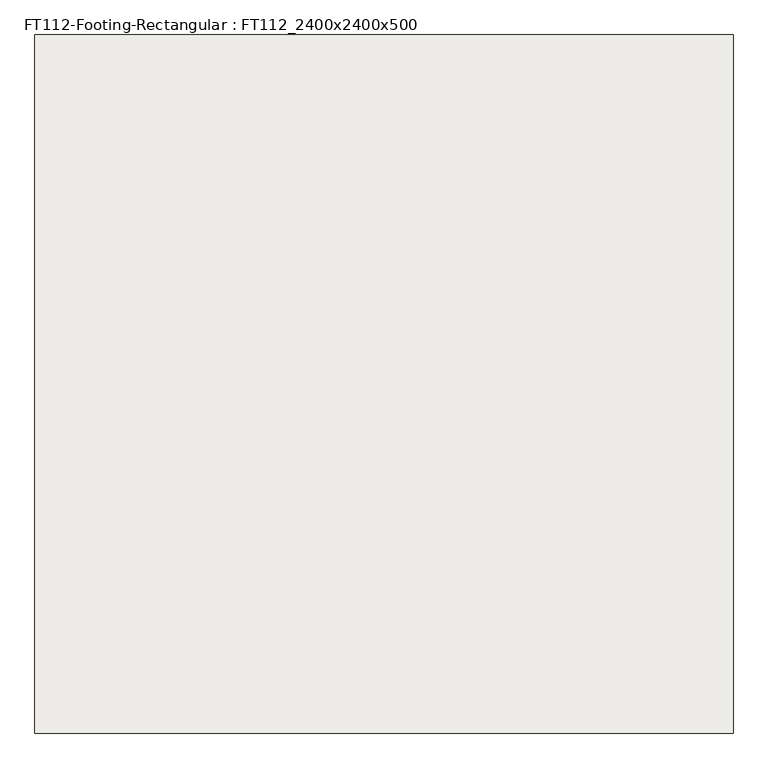
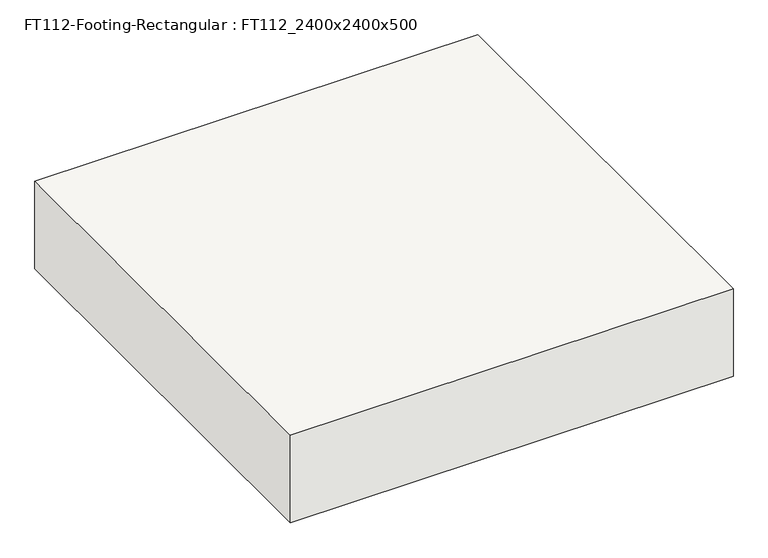
"""IFC4 building model written with IfcOpenShell, lengths in millimetres: slab geometry, FT112-Footing-Rectangular : FT112_2400x2400x500."""

import ifcopenshell
import ifcopenshell.guid

model = None  # the IFC model being written
_history = None  # IfcOwnerHistory: only IFC2X3 demands one
_inside = {}  # id of a spatial element -> (the spatial element, [elements in it])
_under = {}  # id of a project, library or spatial element -> (it, [spatial elements below it])
_declared = {}  # id of a project -> (the project, [libraries it declares])
_typed = {}  # id of a type object -> (the type object, [elements of that type])
_made_of = {}  # id of a material, layer set ... -> (it, [elements and type objects made of it])


def new_model(schema):
    """Start an empty IFC model of exactly this schema.

    Asked for "IFC4X3", IfcOpenShell would pick the latest addendum, in which some entities
    have other attributes; the version numbers below select the first issue.
    IFC2X3 requires an IfcOwnerHistory on every rooted entity: one is made here for all.
    """
    global model, _history
    if schema == "IFC4X3":
        model = ifcopenshell.file(schema_version=(4, 3, 0, 0))
    else:
        model = ifcopenshell.file(schema=schema)
    _inside.clear()
    _under.clear()
    _declared.clear()
    _typed.clear()
    _made_of.clear()
    _history = None
    if model.schema == "IFC2X3":
        org = make("IfcOrganization", Name="unknown")
        user = make(
            "IfcPersonAndOrganization",
            ThePerson=make("IfcPerson", FamilyName="unknown"),
            TheOrganization=org,
        )
        app = make(
            "IfcApplication",
            ApplicationDeveloper=org,
            Version="unknown",
            ApplicationFullName="unknown",
            ApplicationIdentifier="unknown",
        )
        _history = make(
            "IfcOwnerHistory",
            OwningUser=user,
            OwningApplication=app,
            ChangeAction="ADDED",
            CreationDate=0,
        )
    return model


def make(cls, **values):
    """One entity of the class cls with the attributes given. An attribute that is None is left unset."""
    return model.create_entity(
        cls, **{name: value for name, value in values.items() if value is not None}
    )


def rooted(cls, **values):
    """An entity with a GlobalId (a new one), such as an element, a storey or a relation."""
    return make(cls, GlobalId=ifcopenshell.guid.new(), OwnerHistory=_history, **values)


def si_unit(unit_type, name, prefix=None):
    """IfcSIUnit, for example si_unit("LENGTHUNIT", "METRE", prefix="MILLI")."""
    return make("IfcSIUnit", UnitType=unit_type, Prefix=prefix, Name=name)


def assignment(units):
    """IfcUnitAssignment: the units of a project."""
    return None if units is None else make("IfcUnitAssignment", Units=units)


def point(xyz):
    """IfcCartesianPoint."""
    return None if xyz is None else make("IfcCartesianPoint", Coordinates=xyz)


def direction(xyz):
    """IfcDirection."""
    return None if xyz is None else make("IfcDirection", DirectionRatios=xyz)


def frame(location, z_axis=None, x_axis=None):
    """IfcAxis2Placement3D, a coordinate frame: its origin and axes. An axis left out is left unset."""
    return make(
        "IfcAxis2Placement3D",
        Location=point(location),
        Axis=direction(z_axis),
        RefDirection=direction(x_axis),
    )


def origin():
    """The frame at (0, 0, 0) with its axes left unset."""
    return frame((0.0, 0.0, 0.0))


def place(relative_to, where):
    """IfcLocalPlacement: puts the frame where relative to a parent placement (None: the world)."""
    return make(
        "IfcLocalPlacement", PlacementRelTo=relative_to, RelativePlacement=where
    )


def context(
    kind, dimensions, precision=None, world=None, true_north=None, identifier=None
):
    """IfcGeometricRepresentationContext, for example the 3D "Model" context."""
    return make(
        "IfcGeometricRepresentationContext",
        ContextIdentifier=identifier,
        ContextType=kind,
        CoordinateSpaceDimension=dimensions,
        Precision=precision,
        WorldCoordinateSystem=world,
        TrueNorth=true_north,
    )


def project(units=None, contexts=None):
    """IfcProject with its units and contexts."""
    return rooted(
        "IfcProject",
        Name="project",
        RepresentationContexts=contexts,
        UnitsInContext=assignment(units),
    )


def spatial(cls, under=None, at=None, **own):
    """A site, building, storey or space (cls), placed at a placement, below another one or the project."""
    s = rooted(cls, ObjectPlacement=at, **own)
    if under is not None:
        _under.setdefault(under.id(), (under, []))[1].append(s)
    return s


def polyline(points):
    """IfcPolyline through the points."""
    return make("IfcPolyline", Points=[point(p) for p in points])


def outline(outer, holes=None, kind="AREA"):
    """IfcArbitraryClosedProfileDef: a profile drawn as a closed curve; with holes, ...WithVoids."""
    if holes is None:
        return make("IfcArbitraryClosedProfileDef", ProfileType=kind, OuterCurve=outer)
    return make(
        "IfcArbitraryProfileDefWithVoids",
        ProfileType=kind,
        OuterCurve=outer,
        InnerCurves=holes,
    )


def extrude(swept, where, along, depth):
    """IfcExtrudedAreaSolid: the profile swept, set in the frame where, extruded along a direction by depth."""
    return make(
        "IfcExtrudedAreaSolid",
        SweptArea=swept,
        Position=where,
        ExtrudedDirection=direction(along),
        Depth=depth,
    )


def shape(context_of_items, identifier, shape_type, items):
    """IfcShapeRepresentation: the items that make up one representation, for example the "Body"."""
    return make(
        "IfcShapeRepresentation",
        ContextOfItems=context_of_items,
        RepresentationIdentifier=identifier,
        RepresentationType=shape_type,
        Items=items,
    )


def source(mapping_origin, context_of_items, identifier, shape_type, items):
    """IfcRepresentationMap: a shape defined once, which mapped items show again and again."""
    return make(
        "IfcRepresentationMap",
        MappingOrigin=mapping_origin,
        MappedRepresentation=shape(context_of_items, identifier, shape_type, items),
    )


def transform(
    local_origin,
    x_axis=None,
    y_axis=None,
    z_axis=None,
    scale=None,
    scale2=None,
    scale3=None,
    uniform=True,
):
    """IfcCartesianTransformationOperator3D, or its non-uniform kind. x_axis, y_axis, z_axis: its Axis1, 2, 3."""
    if uniform:
        return make(
            "IfcCartesianTransformationOperator3D",
            Axis1=direction(x_axis),
            Axis2=direction(y_axis),
            LocalOrigin=point(local_origin),
            Scale=scale,
            Axis3=direction(z_axis),
        )
    return make(
        "IfcCartesianTransformationOperator3DnonUniform",
        Axis1=direction(x_axis),
        Axis2=direction(y_axis),
        LocalOrigin=point(local_origin),
        Scale=scale,
        Axis3=direction(z_axis),
        Scale2=scale2,
        Scale3=scale3,
    )


def mapped(mapping_source, mapping_target):
    """IfcMappedItem: shows the shape of a source again, moved by a transform."""
    return make(
        "IfcMappedItem", MappingSource=mapping_source, MappingTarget=mapping_target
    )


def made_of(thing, what):
    """Note that an element or type object is made of a material, layer set ...; save() writes the relation."""
    if what is not None:
        _made_of.setdefault(what.id(), (what, []))[1].append(thing)
    return thing


def element(
    cls,
    number,
    at=None,
    inside=None,
    cuts=None,
    type_object=None,
    material=None,
    context=None,
    identifier="Body",
    shape_type=None,
    held_by="IfcProductDefinitionShape",
    body=None,
    shapes=None,
    **own,
):
    """One element of the class cls, such as IfcWall. Its Tag is "e" and its number.

    at: its placement. inside: the storey or other place that contains it. cuts: it is an
    opening in that element (IfcRelVoidsElement). A single representation is given by context,
    identifier, shape_type and body (its items); several are given by shapes. held_by: the class
    of the entity that holds the representations. save() writes the other relations.
    """
    e = rooted(cls, Tag="e%d" % number, ObjectPlacement=at, **own)
    if body is not None:
        shapes = [shape(context, identifier, shape_type, body)]
    if shapes is not None:
        e.Representation = make(held_by, Representations=shapes)
    if inside is not None:
        _inside.setdefault(inside.id(), (inside, []))[1].append(e)
    if cuts is not None:
        rooted(
            "IfcRelVoidsElement", RelatingBuildingElement=cuts, RelatedOpeningElement=e
        )
    if type_object is not None:
        _typed.setdefault(type_object.id(), (type_object, []))[1].append(e)
    return made_of(e, material)


def aggregate(whole, parts):
    """IfcRelAggregates: a whole, such as a stair, and the parts it consists of."""
    return rooted("IfcRelAggregates", RelatingObject=whole, RelatedObjects=parts)


def save(model, path):
    """Write the relations noted so far, then the file.

    IfcRelAggregates (storeys below a building ...), IfcRelContainedInSpatialStructure (elements
    in a storey), IfcRelDefinesByType, IfcRelAssociatesMaterial and IfcRelDeclares: one each for
    every whole, place, type object, material and project.
    """
    for whole, parts in _under.values():
        aggregate(whole, parts)
    for where, things in _inside.values():
        rooted(
            "IfcRelContainedInSpatialStructure",
            RelatedElements=things,
            RelatingStructure=where,
        )
    for kind, things in _typed.values():
        rooted("IfcRelDefinesByType", RelatedObjects=things, RelatingType=kind)
    for what, things in _made_of.values():
        rooted("IfcRelAssociatesMaterial", RelatedObjects=things, RelatingMaterial=what)
    for by, libraries in _declared.values():
        rooted("IfcRelDeclares", RelatingContext=by, RelatedDefinitions=libraries)
    model.write(path)


def ft112_footing_rectangular_ft112_2400x2400x500_5fe39465(model_context):
    return source(origin(), model_context, "Body", "SweptSolid", [
        extrude(outline(polyline([(1200.0, 1200.0), (1200.0, -1200.0), (-1200.0, -1200.0), (-1200.0, 1200.0), (1200.0, 1200.0)])), frame((0.0, 0.0, -500.0), z_axis=(0.0, 0.0, 1.0), x_axis=(1.0, 0.0, 0.0)), (0.0, 0.0, 1.0), 500.0),
    ])


if __name__ == "__main__":
    model = new_model("IFC4")
    model_context = context("Model", 3, world=origin())
    ifc_project = project(units=[si_unit("LENGTHUNIT", "METRE", prefix="MILLI")], contexts=[model_context])
    site = spatial("IfcSite", under=ifc_project)
    building = spatial("IfcBuilding", under=site)
    placement = place(None, origin())
    ft112_footing_rectangular_ft112_2400x2400x500_shape = ft112_footing_rectangular_ft112_2400x2400x500_5fe39465(model_context)
    element("IfcSlab", 1, ObjectType="FT112-Footing-Rectangular : FT112_2400x2400x500", at=placement, inside=building, context=model_context, shape_type="MappedRepresentation", body=[
        mapped(ft112_footing_rectangular_ft112_2400x2400x500_shape, transform((0.0, 0.0, 0.0), x_axis=(1.0, 0.0, 0.0), y_axis=(0.0, 1.0, 0.0), z_axis=(0.0, 0.0, 1.0))),
    ])
    save(model, "model.ifc")

# Revit data of these elements
# Type "FT112-Footing-Rectangular : FT112_2400x2400x500"
#   Description = "UG Shallow Foundation"
#   Width = 2400 mm
#   Length = 2400 mm
#   Foundation Thickness = 500 mm
#   hec_material3 [instance default] = none
#   hec_material2 [instance default] = A03AE056-00001_Bitumen/Bituminous/Asphalt Coating
#   hec_material1 [instance default] = A03AC035-00001_Form Work (3 times in use)_Flat
#   Structural Material [instance default] = A03AC032-00007_Structural Concrete_Type1_25MPa-30Mpa
#   Assembly Code = ""
# Element 1 (IfcSlab, "FT112-Footing-Rectangular : FT112_2400x2400x500")
#   Structural Material = 콘크리트 - 현장타설 콘크리트
#   Materials on its faces: "콘크리트 - 현장타설 콘크리트"
# Materials
#   "A03AE056-00001_Bitumen/Bituminous/Asphalt Coating": class "Generic", colour RGB 17 17 17, transparency 0, Description = "Damp-proofing", W00) Work Master Code = "A03AE056-00001", W01) Work Master_Lv1 = "Concrete Work", W02) Work Master_Lv2 = "Concrete Protective Coating (U/G)", W03) Work Master_Spec.1 = "Bitumen/Bituminous/Asphalt Coating", Cost = 0
#   "A03AC035-00001_Form Work (3 times in use)_Flat": class "Wood", colour RGB 149 120 74, transparency 0, Description = "Plywood", W00) Work Master Code = "A03AC035-00001", W01) Work Master_Lv1 = "Concrete Work", W02) Work Master_Lv2 = "Substructure Work", W03) Work Master_Spec.1 = "Form Work (3 times in use)", W04) Work Master_Spec.2 = "Flat Form", W05) Work Master_Spec.3 = "Dressed Lumber, Plywood or Steel Form(Wood Planks are not Allowed) incl. Chamfer", Cost = 0
#   "A03AC032-00007_Structural Concrete_Type1_25MPa-30Mpa": class "Concrete", colour RGB 176 176 176, transparency 0, Keynote = "09910.A1", Description = "Reinf. Conc.", W00) Work Master Code = "A03AC032-00007", W01) Work Master_Lv1 = "Concrete Work", W02) Work Master_Lv2 = "Substructure Work", W03) Work Master_Spec.1 = "Structural Concrete", W04) Work Master_Spec.2 = "Cement Type-1", W05) Work Master_Spec.3 = "25MPa < F'c (Cylinder Strength) ≤ 30MPa", Cost = 0
#   "콘크리트 - 현장타설 콘크리트": class "콘크리트", colour RGB 192 192 192, transparency 0
